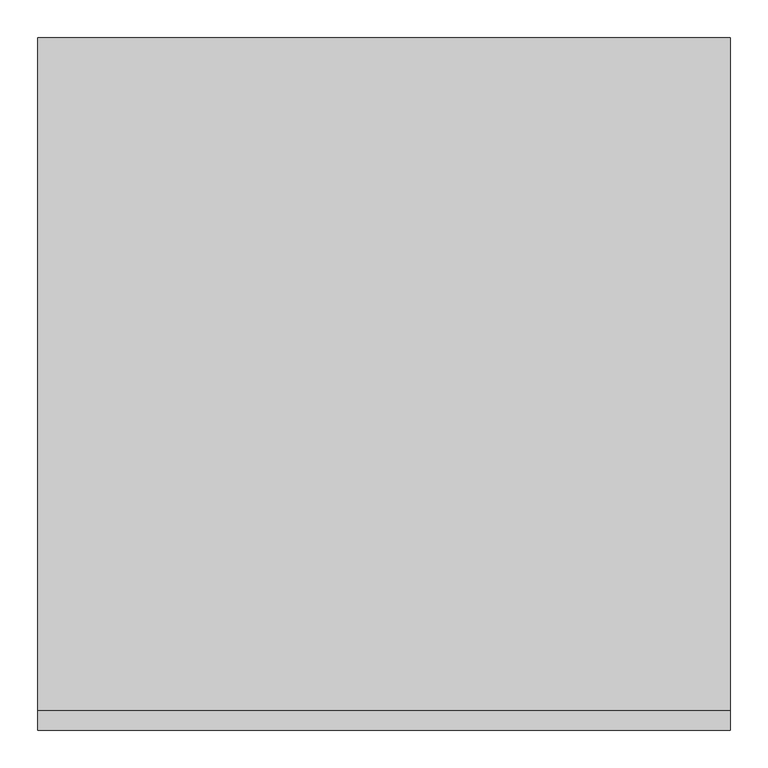
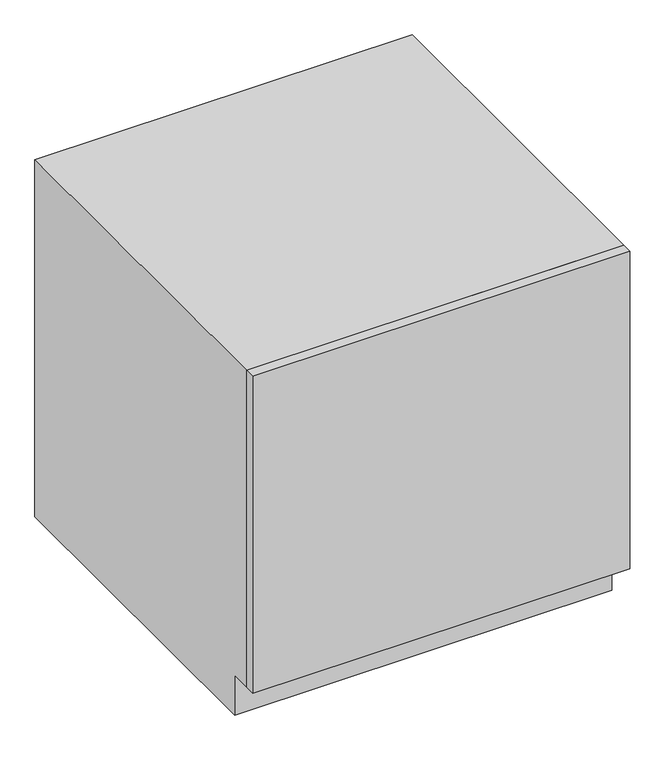
"""IFC4 building model written with IfcOpenShell, lengths in millimetres: furniture geometry, OD_CW_Base Cabinet : OD_CW_Base Cabinet."""

from ifc_helpers import new_model, si_unit, frame, origin, place, context, project, spatial, polyline, outline, extrude, source, transform, mapped, element, save


def furniture_676407f5(model_context):
    return source(origin(), model_context, "Body", "SweptSolid", [
        extrude(outline(polyline([(18.7377049, -279.4), (933.1377049, -279.4), (933.1377049, -304.8), (18.7377049, -304.8), (18.7377049, -279.4)])), frame((0.0, 0.0, 101.6), z_axis=(0.0, 0.0, 1.0), x_axis=(1.0, 0.0, 0.0)), (0.0, 0.0, 1.0), 812.8),
        extrude(outline(polyline([(-279.4, 914.4), (609.6, 914.4), (609.6, 0.0), (-228.6, 0.0), (-228.6, 101.6), (-279.4, 101.6), (-279.4, 914.4)])), frame((18.7377049, 0.0, 0.0), z_axis=(1.0, 0.0, 0.0), x_axis=(0.0, 1.0, 0.0)), (0.0, 0.0, 1.0), 914.4),
    ])


if __name__ == "__main__":
    model = new_model("IFC4")
    model_context = context("Model", 3, world=origin())
    ifc_project = project(units=[si_unit("LENGTHUNIT", "METRE", prefix="MILLI")], contexts=[model_context])
    site = spatial("IfcSite", under=ifc_project)
    building = spatial("IfcBuilding", under=site)
    placement = place(None, origin())
    furniture_shape = furniture_676407f5(model_context)
    element("IfcFurniture", 1, ObjectType="OD_CW_Base Cabinet : OD_CW_Base Cabinet", at=placement, inside=building, context=model_context, shape_type="MappedRepresentation", body=[
        mapped(furniture_shape, transform((0.0, 0.0, 0.0), x_axis=(1.0, 0.0, 0.0), y_axis=(0.0, 1.0, 0.0), z_axis=(0.0, 0.0, 1.0))),
    ])
    save(model, "model.ifc")

# Revit data of these elements
# Type "OD_CW_Base Cabinet : OD_CW_Base Cabinet"
#   OD_CW_Width [instance default] = 2' - 10"
#   OD_CW_Length [instance default] = 8' - 0"
#   OD_CW_Height [instance default] = 2' - 3"
#   Depth = 2' - 0"
#   Height = 3' - 0"
#   Width = 4' - 0"
#   OD_CW_Material_Front Panel [instance default] = none
#   OD_CW_Material_Body [instance default] = none
# Element 1 (IfcFurniture, "OD_CW_Base Cabinet : OD_CW_Base Cabinet")
#   OD_CW_Width = 3' - 0"
#   OD_CW_Length = 3' - 0"
#   OD_CW_Height = 3' - 0"
#   OD_CW_Material_Body = WORKTOP FREEZER - STEAM TABLES ON TOP
#   Materials on its faces: "WORKTOP FREEZER - STEAM TABLES ON TOP", "CASEWORK"
# Materials
#   "WORKTOP FREEZER - STEAM TABLES ON TOP": class "Generic", colour RGB 187 187 187, transparency 0, Cost = 0
#   "CASEWORK": class "Generic", colour RGB 181 181 181, transparency 0, Cost = 0
